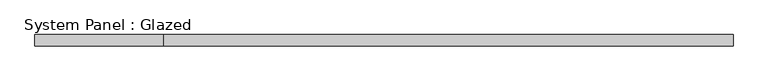
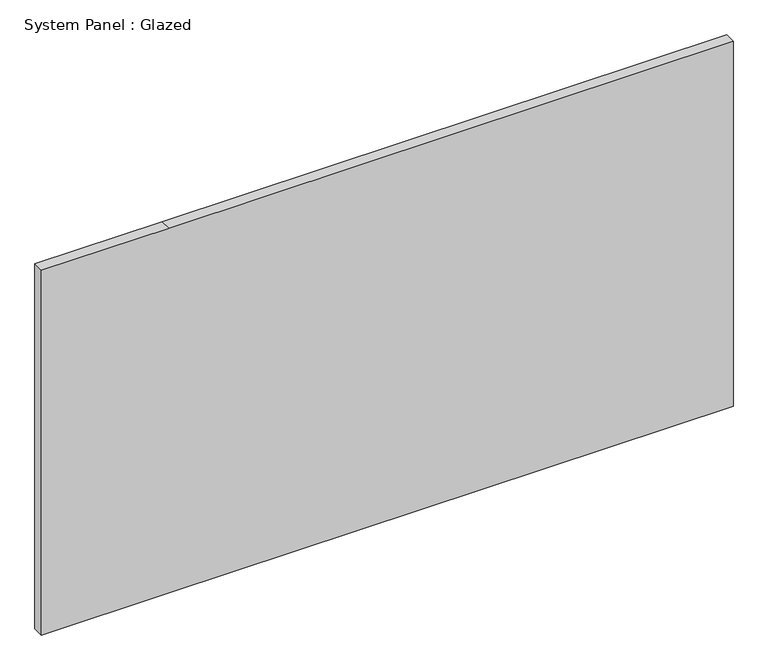
"""IFC4 building model written with IfcOpenShell, lengths in millimetres: plate geometry, System Panel : Glazed."""

from ifc_helpers import new_model, si_unit, frame, origin, place, context, project, spatial, polyline, outline, extrude, source, transform, mapped, element, save


def system_panel_glazed_c6b886e5(model_context):
    return source(origin(), model_context, "Body", "SweptSolid", [
        extrude(outline(polyline([(0.0, -774.7), (0.0, -488.95), (0.0, 774.7), (863.6, 774.7), (863.6, -488.95), (863.6, -774.7), (0.0, -774.7)])), frame((0.0, 19.05, 0.0), z_axis=(0.0, 1.0, 0.0), x_axis=(0.0, 0.0, 1.0)), (0.0, 0.0, 1.0), 25.4),
    ])


if __name__ == "__main__":
    model = new_model("IFC4")
    model_context = context("Model", 3, world=origin())
    ifc_project = project(units=[si_unit("LENGTHUNIT", "METRE", prefix="MILLI")], contexts=[model_context])
    site = spatial("IfcSite", under=ifc_project)
    building = spatial("IfcBuilding", under=site)
    placement = place(None, origin())
    system_panel_glazed_shape = system_panel_glazed_c6b886e5(model_context)
    element("IfcPlate", 1, ObjectType="System Panel : Glazed", at=placement, inside=building, context=model_context, shape_type="MappedRepresentation", body=[
        mapped(system_panel_glazed_shape, transform((0.0, 0.0, 0.0), x_axis=(1.0, 0.0, 0.0), y_axis=(0.0, 1.0, 0.0), z_axis=(0.0, 0.0, 1.0))),
    ])
    save(model, "model.ifc")

# Revit data of these elements
# Element 1 (IfcPlate, "System Panel : Glazed")
#   Materials on its faces: "Glass"
# Materials
#   "Glass": class "Glass", colour RGB 0 128 192, transparency 0.75, Cost = 0
